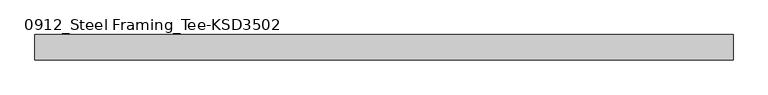
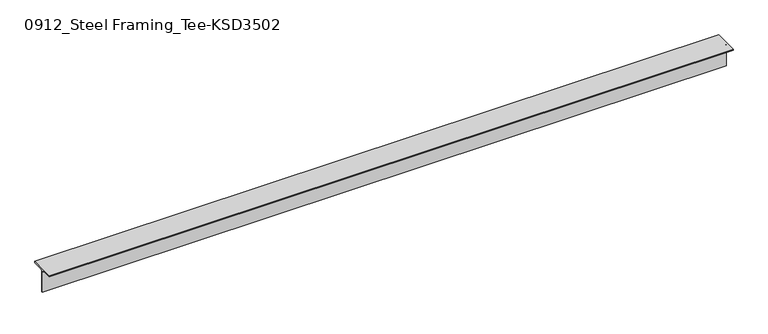
"""IFC4 building model written with IfcOpenShell, lengths in millimetres: member geometry, 0912_Steel Framing_Tee-KSD3502 : H_SB_ASB_CT-150x150x6.5x9."""

from ifc_helpers import new_model, si_unit, point, frame, frame_2d, origin, place, context, project, spatial, polyline, circle_curve, trimmed, segment, composite_curve, outline, extrude, source, transform, mapped, element, save


def member_0912_steel_framing_tee_ksd3502_6142c849(model_context):
    return source(origin(), model_context, "Body", "SweptSolid", [
        extrude(outline(composite_curve([segment(polyline([(-75.0, 75.0), (75.0, 75.0), (75.0, 66.0), (16.25, 66.0)]), True, "CONTINUOUS"), segment(trimmed(circle_curve(frame_2d((16.25, 53.0)), 13.0), [point((16.25, 66.0))], [point((3.25, 53.0))], True, "CARTESIAN"), True, "CONTINUOUS"), segment(polyline([(3.25, 53.0), (3.25, -75.0), (-3.25, -75.0), (-3.25, 53.0)]), True, "CONTINUOUS"), segment(trimmed(circle_curve(frame_2d((-16.25, 53.0)), 13.0), [point((-3.25, 53.0))], [point((-16.25, 66.0))], True, "CARTESIAN"), True, "CONTINUOUS"), segment(polyline([(-16.25, 66.0), (-75.0, 66.0), (-75.0, 75.0)]), True, "CONTINUOUS")], self_intersect=False)), frame((-2106.25, 0.0, 0.0), z_axis=(1.0, 0.0, 0.0), x_axis=(0.0, 1.0, 0.0)), (0.0, 0.0, 1.0), 4152.3),
    ])


if __name__ == "__main__":
    model = new_model("IFC4")
    model_context = context("Model", 3, world=origin())
    ifc_project = project(units=[si_unit("LENGTHUNIT", "METRE", prefix="MILLI")], contexts=[model_context])
    site = spatial("IfcSite", under=ifc_project)
    building = spatial("IfcBuilding", under=site)
    placement = place(None, origin())
    member_0912_steel_framing_tee_ksd3502_shape = member_0912_steel_framing_tee_ksd3502_6142c849(model_context)
    element("IfcMember", 1, ObjectType="0912_Steel Framing_Tee-KSD3502 : H_SB_ASB_CT-150x150x6.5x9", at=placement, inside=building, context=model_context, shape_type="MappedRepresentation", body=[
        mapped(member_0912_steel_framing_tee_ksd3502_shape, transform((0.0, 0.0, 0.0), x_axis=(1.0, 0.0, 0.0), y_axis=(0.0, 1.0, 0.0), z_axis=(0.0, 0.0, 1.0))),
    ])
    save(model, "model.ifc")

# Revit data of these elements
# Type "0912_Steel Framing_Tee-KSD3502 : H_SB_ASB_CT-150x150x6.5x9"
#   H_WM Code_1 = "S01AA003-00001 | Main Steel Structure Fabrication Work | Shelter/Building | Light Steel - Standard (30KG/M>Weight) | Material: (   )"
#   H_WM Code_2 = "S03AA029-00001 | Main Steel Structure Erection Work | Shelter/Building | Light Steel (30KG/M>Weight) | Material: (   )"
#   H_WM Code_3 = "S01AA010-00001 | Main Steel Structure Fabrication Work | Shelter/Building | Steel Painting/Coating | for Non-Fireproofed Steel Surface, Surface Preparation, Primer, Second & Final Coat | Material: (   )"
#   H_Q'ty Cal Type Tag = "SB-Q2"
#   Width = 15.0 cm
#   Web Thickness = 0.65 cm
#   Web Fillet = 1.3 cm
#   Section Area = 23.39 cm²
#   Perimeter = 0.60 m²/m
#   Nominal Weight = 18.40 kgf/m
#   Height = 15.0 cm
#   Flange Thickness = 0.9 cm
#   Centroid Vertical = 7.5 cm
#   Centroid Horizontal = 7.5 cm
#   Length [instance default] = 1.5000 m
#   Structural Material [instance default] = Steel, 45-345
#   Warping Constant = (empty or 0)
#   Torsional Moment of Inertia = 0
#   Section Name Key = ""
#   Plastic Modulus weak axis = 0
#   Plastic Modulus strong axis = 0
#   Moment of Inertia weak axis = 0
#   Moment of Inertia strong axis = 0
#   Elastic Modulus weak axis = 0
#   Elastic Modulus strong axis = 0
#   Bolt Spacing = 0
#   Assembly Code = ""
# Element 1 (IfcMember, "0912_Steel Framing_Tee-KSD3502 : H_SB_ASB_CT-150x150x6.5x9")
#   Structural Material = none
# Materials
#   "Steel, 45-345": class "Metal", colour RGB 189 187 185, transparency 0, Description = "Steel 345 MPa", Cost = 0
